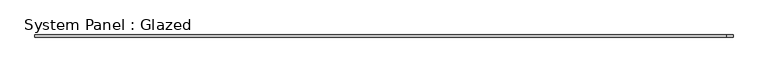
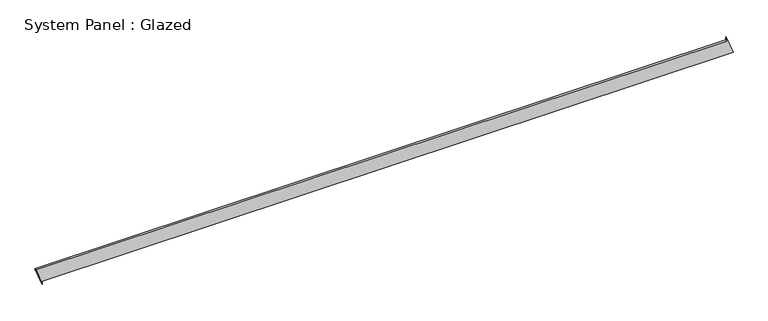
"""IFC4 building model written with IfcOpenShell, lengths in millimetres: plate geometry, System Panel : Glazed."""

from ifc_helpers import new_model, si_unit, frame, origin, place, context, project, spatial, polyline, outline, extrude, source, transform, mapped, element, save


def system_panel_glazed_f276d973(model_context):
    return source(origin(), model_context, "Body", "SweptSolid", [
        extrude(outline(polyline([(0.0, -3957.2941299), (35.3553391, -3957.2941299), (35.3553391, 4028.0649835), (233.5239524, 3956.4980838), (198.1686134, 3956.4965613), (198.5124481, -4028.0649835), (0.0, -3957.2941299)])), frame((0.0, -49.5, 0.0), z_axis=(0.0, 1.0, 0.0), x_axis=(0.0, 0.0, 1.0)), (0.0, 0.0, 1.0), 25.0),
    ])


if __name__ == "__main__":
    model = new_model("IFC4")
    model_context = context("Model", 3, world=origin())
    ifc_project = project(units=[si_unit("LENGTHUNIT", "METRE", prefix="MILLI")], contexts=[model_context])
    site = spatial("IfcSite", under=ifc_project)
    building = spatial("IfcBuilding", under=site)
    placement = place(None, origin())
    system_panel_glazed_shape = system_panel_glazed_f276d973(model_context)
    element("IfcPlate", 1, ObjectType="System Panel : Glazed", at=placement, inside=building, context=model_context, shape_type="MappedRepresentation", body=[
        mapped(system_panel_glazed_shape, transform((0.0, 0.0, 0.0), x_axis=(1.0, 0.0, 0.0), y_axis=(0.0, 1.0, 0.0), z_axis=(0.0, 0.0, 1.0))),
    ])
    save(model, "model.ifc")

# Revit data of these elements
# Element 1 (IfcPlate, "System Panel : Glazed")
#   Materials on its faces: "Glass"
# Materials
#   "Glass": class "Glass", colour RGB 218 227 224, transparency 0.85, Description = "Soda Lime Glass", Cost = 0
